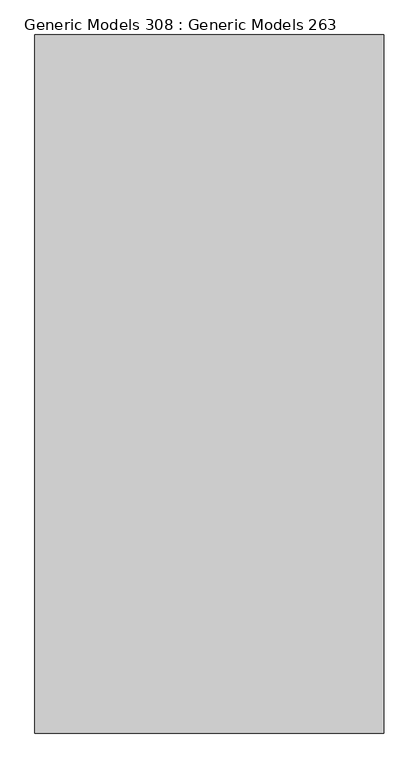
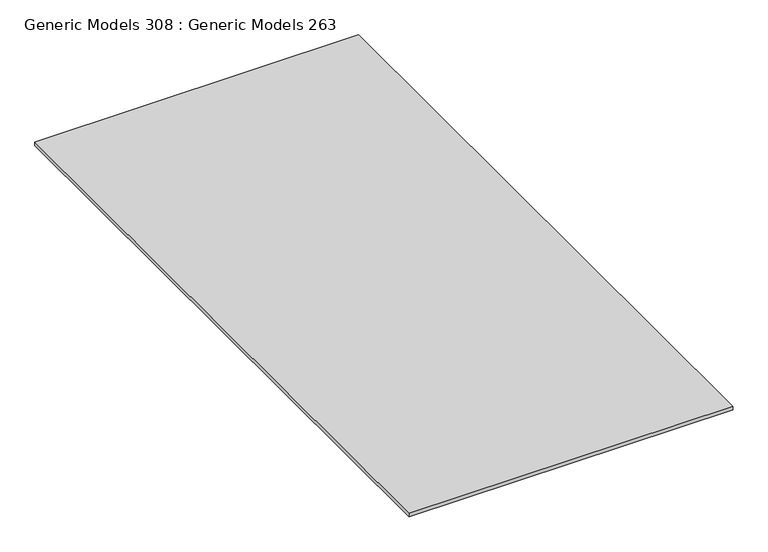
"""IFC4 building model written with IfcOpenShell, lengths in millimetres: proxy geometry, Generic Models 308 : Generic Models 263."""

from ifc_helpers import new_model, si_unit, origin, origin_with_axes, place, context, project, spatial, polyline, outline, extrude, source, transform, mapped, element, save


def generic_models_308_generic_models_263_61ecfa5a(model_context):
    return source(origin(), model_context, "Body", "SweptSolid", [
        extrude(outline(polyline([(95516.9797726, -94.4486541), (94907.3797726, -94.4486541), (94907.3797726, 1124.7513459), (95516.9797726, 1124.7513459), (95516.9797726, -94.4486541)])), origin_with_axes(), (0.0, 0.0, 1.0), 7.0017153),
    ])


if __name__ == "__main__":
    model = new_model("IFC4")
    model_context = context("Model", 3, world=origin())
    ifc_project = project(units=[si_unit("LENGTHUNIT", "METRE", prefix="MILLI")], contexts=[model_context])
    site = spatial("IfcSite", under=ifc_project)
    building = spatial("IfcBuilding", under=site)
    placement = place(None, origin())
    generic_models_308_generic_models_263_shape = generic_models_308_generic_models_263_61ecfa5a(model_context)
    element("IfcBuildingElementProxy", 1, Name="Generic Models 308 : Generic Models 263", ObjectType="Generic Models 308 : Generic Models 263", at=placement, inside=building, context=model_context, shape_type="MappedRepresentation", body=[
        mapped(generic_models_308_generic_models_263_shape, transform((0.0, 0.0, 0.0), x_axis=(1.0, 0.0, 0.0), y_axis=(0.0, 1.0, 0.0), z_axis=(0.0, 0.0, 1.0))),
    ])
    save(model, "model.ifc")

# Revit data of these elements
# Element 1 (IfcBuildingElementProxy, "Generic Models 308 : Generic Models 263")
#   Materials on its faces: "MEDIUM BROOM FINISH"
# Materials
#   "MEDIUM BROOM FINISH": class "Miscellaneous", colour RGB 44 44 44, transparency 0, Cost = 0
